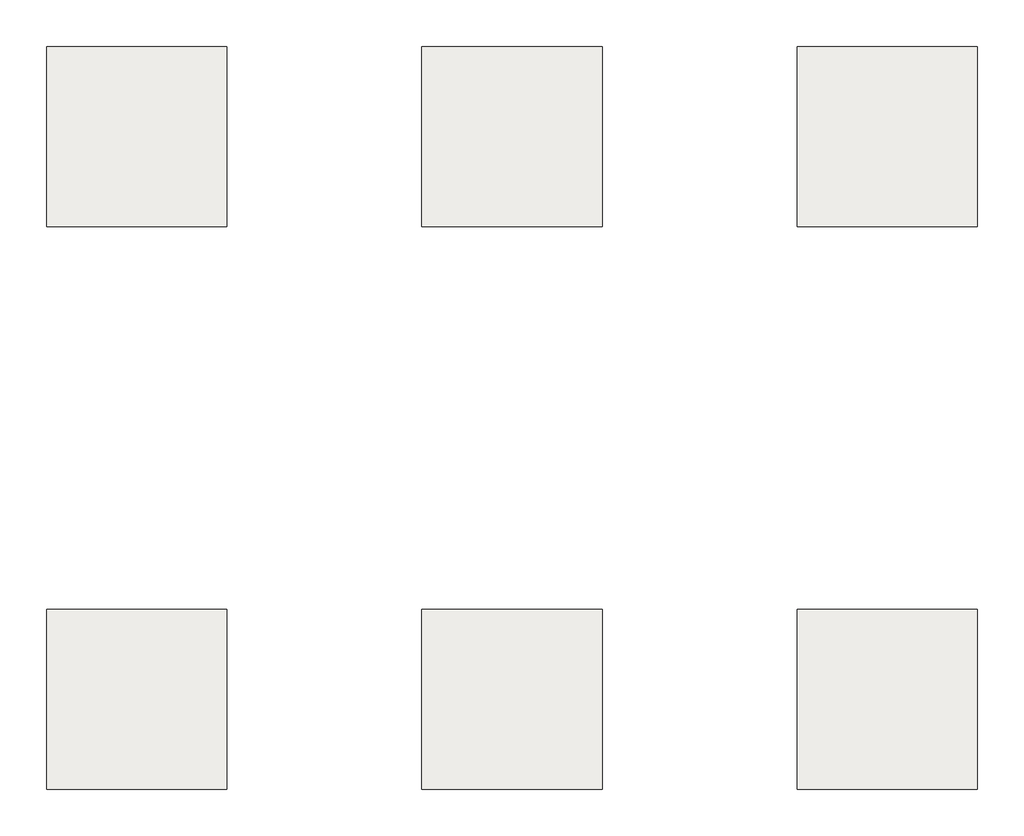
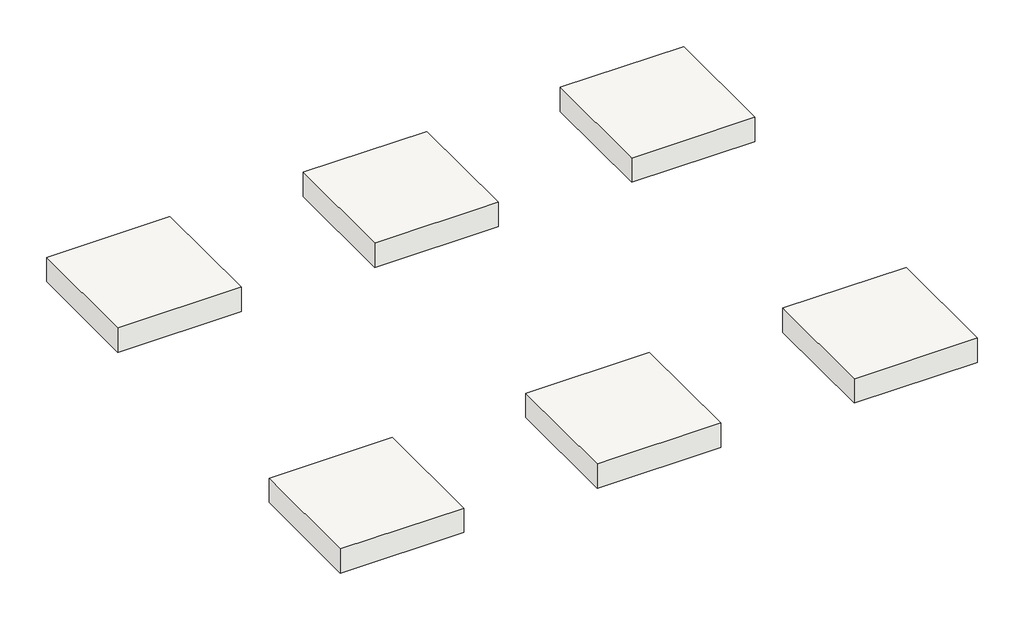
# Not in any storey: 6 slabs.
"""IFC4 building model written with IfcOpenShell, lengths in millimetres."""

import ifcopenshell
import ifcopenshell.guid

model = None  # the IFC model being written
_history = None  # IfcOwnerHistory: only IFC2X3 demands one
_inside = {}  # id of a spatial element -> (the spatial element, [elements in it])
_under = {}  # id of a project, library or spatial element -> (it, [spatial elements below it])
_declared = {}  # id of a project -> (the project, [libraries it declares])
_typed = {}  # id of a type object -> (the type object, [elements of that type])
_made_of = {}  # id of a material, layer set ... -> (it, [elements and type objects made of it])


def new_model(schema):
    """Start an empty IFC model of exactly this schema.

    Asked for "IFC4X3", IfcOpenShell would pick the latest addendum, in which some entities
    have other attributes; the version numbers below select the first issue.
    IFC2X3 requires an IfcOwnerHistory on every rooted entity: one is made here for all.
    """
    global model, _history
    if schema == "IFC4X3":
        model = ifcopenshell.file(schema_version=(4, 3, 0, 0))
    else:
        model = ifcopenshell.file(schema=schema)
    _inside.clear()
    _under.clear()
    _declared.clear()
    _typed.clear()
    _made_of.clear()
    _history = None
    if model.schema == "IFC2X3":
        org = make("IfcOrganization", Name="unknown")
        user = make(
            "IfcPersonAndOrganization",
            ThePerson=make("IfcPerson", FamilyName="unknown"),
            TheOrganization=org,
        )
        app = make(
            "IfcApplication",
            ApplicationDeveloper=org,
            Version="unknown",
            ApplicationFullName="unknown",
            ApplicationIdentifier="unknown",
        )
        _history = make(
            "IfcOwnerHistory",
            OwningUser=user,
            OwningApplication=app,
            ChangeAction="ADDED",
            CreationDate=0,
        )
    return model


def make(cls, **values):
    """One entity of the class cls with the attributes given. An attribute that is None is left unset."""
    return model.create_entity(
        cls, **{name: value for name, value in values.items() if value is not None}
    )


def rooted(cls, **values):
    """An entity with a GlobalId (a new one), such as an element, a storey or a relation."""
    return make(cls, GlobalId=ifcopenshell.guid.new(), OwnerHistory=_history, **values)


def si_unit(unit_type, name, prefix=None):
    """IfcSIUnit, for example si_unit("LENGTHUNIT", "METRE", prefix="MILLI")."""
    return make("IfcSIUnit", UnitType=unit_type, Prefix=prefix, Name=name)


def assignment(units):
    """IfcUnitAssignment: the units of a project."""
    return None if units is None else make("IfcUnitAssignment", Units=units)


def point(xyz):
    """IfcCartesianPoint."""
    return None if xyz is None else make("IfcCartesianPoint", Coordinates=xyz)


def direction(xyz):
    """IfcDirection."""
    return None if xyz is None else make("IfcDirection", DirectionRatios=xyz)


def frame(location, z_axis=None, x_axis=None):
    """IfcAxis2Placement3D, a coordinate frame: its origin and axes. An axis left out is left unset."""
    return make(
        "IfcAxis2Placement3D",
        Location=point(location),
        Axis=direction(z_axis),
        RefDirection=direction(x_axis),
    )


def origin():
    """The frame at (0, 0, 0) with its axes left unset."""
    return frame((0.0, 0.0, 0.0))


def place(relative_to, where):
    """IfcLocalPlacement: puts the frame where relative to a parent placement (None: the world)."""
    return make(
        "IfcLocalPlacement", PlacementRelTo=relative_to, RelativePlacement=where
    )


def context(
    kind, dimensions, precision=None, world=None, true_north=None, identifier=None
):
    """IfcGeometricRepresentationContext, for example the 3D "Model" context."""
    return make(
        "IfcGeometricRepresentationContext",
        ContextIdentifier=identifier,
        ContextType=kind,
        CoordinateSpaceDimension=dimensions,
        Precision=precision,
        WorldCoordinateSystem=world,
        TrueNorth=true_north,
    )


def project(units=None, contexts=None):
    """IfcProject with its units and contexts."""
    return rooted(
        "IfcProject",
        Name="project",
        RepresentationContexts=contexts,
        UnitsInContext=assignment(units),
    )


def spatial(cls, under=None, at=None, **own):
    """A site, building, storey or space (cls), placed at a placement, below another one or the project."""
    s = rooted(cls, ObjectPlacement=at, **own)
    if under is not None:
        _under.setdefault(under.id(), (under, []))[1].append(s)
    return s


def polyline(points):
    """IfcPolyline through the points."""
    return make("IfcPolyline", Points=[point(p) for p in points])


def outline(outer, holes=None, kind="AREA"):
    """IfcArbitraryClosedProfileDef: a profile drawn as a closed curve; with holes, ...WithVoids."""
    if holes is None:
        return make("IfcArbitraryClosedProfileDef", ProfileType=kind, OuterCurve=outer)
    return make(
        "IfcArbitraryProfileDefWithVoids",
        ProfileType=kind,
        OuterCurve=outer,
        InnerCurves=holes,
    )


def extrude(swept, where, along, depth):
    """IfcExtrudedAreaSolid: the profile swept, set in the frame where, extruded along a direction by depth."""
    return make(
        "IfcExtrudedAreaSolid",
        SweptArea=swept,
        Position=where,
        ExtrudedDirection=direction(along),
        Depth=depth,
    )


def shape(context_of_items, identifier, shape_type, items):
    """IfcShapeRepresentation: the items that make up one representation, for example the "Body"."""
    return make(
        "IfcShapeRepresentation",
        ContextOfItems=context_of_items,
        RepresentationIdentifier=identifier,
        RepresentationType=shape_type,
        Items=items,
    )


def source(mapping_origin, context_of_items, identifier, shape_type, items):
    """IfcRepresentationMap: a shape defined once, which mapped items show again and again."""
    return make(
        "IfcRepresentationMap",
        MappingOrigin=mapping_origin,
        MappedRepresentation=shape(context_of_items, identifier, shape_type, items),
    )


def transform(
    local_origin,
    x_axis=None,
    y_axis=None,
    z_axis=None,
    scale=None,
    scale2=None,
    scale3=None,
    uniform=True,
):
    """IfcCartesianTransformationOperator3D, or its non-uniform kind. x_axis, y_axis, z_axis: its Axis1, 2, 3."""
    if uniform:
        return make(
            "IfcCartesianTransformationOperator3D",
            Axis1=direction(x_axis),
            Axis2=direction(y_axis),
            LocalOrigin=point(local_origin),
            Scale=scale,
            Axis3=direction(z_axis),
        )
    return make(
        "IfcCartesianTransformationOperator3DnonUniform",
        Axis1=direction(x_axis),
        Axis2=direction(y_axis),
        LocalOrigin=point(local_origin),
        Scale=scale,
        Axis3=direction(z_axis),
        Scale2=scale2,
        Scale3=scale3,
    )


def mapped(mapping_source, mapping_target):
    """IfcMappedItem: shows the shape of a source again, moved by a transform."""
    return make(
        "IfcMappedItem", MappingSource=mapping_source, MappingTarget=mapping_target
    )


def made_of(thing, what):
    """Note that an element or type object is made of a material, layer set ...; save() writes the relation."""
    if what is not None:
        _made_of.setdefault(what.id(), (what, []))[1].append(thing)
    return thing


def element(
    cls,
    number,
    at=None,
    inside=None,
    cuts=None,
    type_object=None,
    material=None,
    context=None,
    identifier="Body",
    shape_type=None,
    held_by="IfcProductDefinitionShape",
    body=None,
    shapes=None,
    **own,
):
    """One element of the class cls, such as IfcWall. Its Tag is "e" and its number.

    at: its placement. inside: the storey or other place that contains it. cuts: it is an
    opening in that element (IfcRelVoidsElement). A single representation is given by context,
    identifier, shape_type and body (its items); several are given by shapes. held_by: the class
    of the entity that holds the representations. save() writes the other relations.
    """
    e = rooted(cls, Tag="e%d" % number, ObjectPlacement=at, **own)
    if body is not None:
        shapes = [shape(context, identifier, shape_type, body)]
    if shapes is not None:
        e.Representation = make(held_by, Representations=shapes)
    if inside is not None:
        _inside.setdefault(inside.id(), (inside, []))[1].append(e)
    if cuts is not None:
        rooted(
            "IfcRelVoidsElement", RelatingBuildingElement=cuts, RelatedOpeningElement=e
        )
    if type_object is not None:
        _typed.setdefault(type_object.id(), (type_object, []))[1].append(e)
    return made_of(e, material)


def aggregate(whole, parts):
    """IfcRelAggregates: a whole, such as a stair, and the parts it consists of."""
    return rooted("IfcRelAggregates", RelatingObject=whole, RelatedObjects=parts)


def save(model, path):
    """Write the relations noted so far, then the file.

    IfcRelAggregates (storeys below a building ...), IfcRelContainedInSpatialStructure (elements
    in a storey), IfcRelDefinesByType, IfcRelAssociatesMaterial and IfcRelDeclares: one each for
    every whole, place, type object, material and project.
    """
    for whole, parts in _under.values():
        aggregate(whole, parts)
    for where, things in _inside.values():
        rooted(
            "IfcRelContainedInSpatialStructure",
            RelatedElements=things,
            RelatingStructure=where,
        )
    for kind, things in _typed.values():
        rooted("IfcRelDefinesByType", RelatedObjects=things, RelatingType=kind)
    for what, things in _made_of.values():
        rooted("IfcRelAssociatesMaterial", RelatedObjects=things, RelatingMaterial=what)
    for by, libraries in _declared.values():
        rooted("IfcRelDeclares", RelatingContext=by, RelatedDefinitions=libraries)
    model.write(path)


def foundation_rectangular_non_pile_5fe39465(model_context):
    return source(origin(), model_context, "Body", "SweptSolid", [
        extrude(outline(polyline([(1200.0, 1200.0), (1200.0, -1200.0), (-1200.0, -1200.0), (-1200.0, 1200.0), (1200.0, 1200.0)])), frame((0.0, 0.0, -500.0), z_axis=(0.0, 0.0, 1.0), x_axis=(1.0, 0.0, 0.0)), (0.0, 0.0, 1.0), 500.0),
    ])


model = new_model("IFC4")

# Units and contexts
model_context = context("Model", 3, world=origin())
ifc_project = project(units=[si_unit("LENGTHUNIT", "METRE", prefix="MILLI")], contexts=[model_context])

# Site, building
site = spatial("IfcSite", under=ifc_project)
building = spatial("IfcBuilding", under=site)

# Slabs
placement = place(None, origin())
element("IfcSlab", 1, ObjectType="Foundation Rectangular (Non-Pile) : H_SF_ACF_W2400xL2400xT500", at=placement, inside=building, context=model_context, shape_type="SweptSolid", body=[
    extrude(outline(polyline([(11200.0, 22199.5208589), (11200.0, 19799.5208589), (8800.0, 19799.5208589), (8800.0, 22199.5208589), (11200.0, 22199.5208589)])), frame((0.0, 0.0, -1800.0), z_axis=(0.0, 0.0, 1.0), x_axis=(1.0, 0.0, 0.0)), (0.0, 0.0, 1.0), 500.0),
])
element("IfcSlab", 2, ObjectType="Foundation Rectangular (Non-Pile) : H_SF_ACF_W2400xL2400xT500", at=placement, inside=building, context=model_context, shape_type="SweptSolid", body=[
    extrude(outline(polyline([(6200.0, 22199.5208589), (6200.0, 19799.5208589), (3800.0, 19799.5208589), (3800.0, 22199.5208589), (6200.0, 22199.5208589)])), frame((0.0, 0.0, -1800.0), z_axis=(0.0, 0.0, 1.0), x_axis=(1.0, 0.0, 0.0)), (0.0, 0.0, 1.0), 500.0),
])
element("IfcSlab", 3, ObjectType="Foundation Rectangular (Non-Pile) : H_SF_ACF_W2400xL2400xT500", at=placement, inside=building, context=model_context, shape_type="SweptSolid", body=[
    extrude(outline(polyline([(1200.0, 22199.5208589), (1200.0, 19799.5208589), (-1200.0, 19799.5208589), (-1200.0, 22199.5208589), (1200.0, 22199.5208589)])), frame((0.0, 0.0, -1800.0), z_axis=(0.0, 0.0, 1.0), x_axis=(1.0, 0.0, 0.0)), (0.0, 0.0, 1.0), 500.0),
])
element("IfcSlab", 4, ObjectType="Foundation Rectangular (Non-Pile) : H_SF_ACF_W2400xL2400xT500", at=placement, inside=building, context=model_context, shape_type="SweptSolid", body=[
    extrude(outline(polyline([(1200.0, 14699.5208589), (1200.0, 12299.5208589), (-1200.0, 12299.5208589), (-1200.0, 14699.5208589), (1200.0, 14699.5208589)])), frame((0.0, 0.0, -1800.0), z_axis=(0.0, 0.0, 1.0), x_axis=(1.0, 0.0, 0.0)), (0.0, 0.0, 1.0), 500.0),
])
foundation_rectangular_non_pile_shape = foundation_rectangular_non_pile_5fe39465(model_context)
element("IfcSlab", 5, ObjectType="Foundation Rectangular (Non-Pile) : H_SF_ACF_W2400xL2400xT500", at=placement, inside=building, context=model_context, shape_type="MappedRepresentation", body=[
    mapped(foundation_rectangular_non_pile_shape, transform((5000.0, 13499.5208589, -1300.0), x_axis=(1.0, 0.0, 0.0), y_axis=(0.0, 1.0, 0.0), z_axis=(0.0, 0.0, 1.0))),
])
element("IfcSlab", 6, ObjectType="Foundation Rectangular (Non-Pile) : H_SF_ACF_W2400xL2400xT500", at=placement, inside=building, context=model_context, shape_type="MappedRepresentation", body=[
    mapped(foundation_rectangular_non_pile_shape, transform((10000.0, 13499.5208589, -1300.0), x_axis=(1.0, 0.0, 0.0), y_axis=(0.0, 1.0, 0.0), z_axis=(0.0, 0.0, 1.0))),
])

save(model, "model.ifc")

# Revit data of these elements
# Project information
#   Building Name = "MAIN GATE SECURITY BUILDING"
#   Project Status = "Project Status"
#   Client Name = "현대엔지니어링"
#   Project Address = "서울시 종로구 율곡로 75(계동)"
#   Project Name = "Therma Visayas Energy Project"
#   Project Number = "-"
# Grids (mm)
#   "A": line (0, 24502.793) -> (0, 11308.625)
#   "B": line (5000, 24502.793) -> (5000, 11308.625)
#   "C": line (10000, 24502.793) -> (10000, 11308.625)
#   "1": line (-3860.098, 13499.521) -> (12441.468, 13499.521)
#   "2": line (-3860.098, 20999.521) -> (12441.468, 20999.521)
# Type "Foundation Rectangular (Non-Pile) : H_SF_ACF_W2400xL2400xT500"
#   Top bar = "D25@300"
#   Description = "UG Shallow Foundation"
#   Bottom bar = "D20@300"
#   Width = 2400 mm
#   Length = 2400 mm
#   Foundation Thickness = 500 mm
#   Structural Material [instance default] = A03AC032-00007_Structural Concrete_Type1_25MPa-30Mpa
#   Assembly Code = ""
# Elements 1, 2, 3, 4, 5, 6 (IfcSlab, "Foundation Rectangular (Non-Pile) : H_SF_ACF_W2400xL2400xT500")
#   Comments = ""
#   Mark = "F1"
#   Structural Material = A03AC032-00007_Structural Concrete_Type1_25MPa-30Mpa
#   Phase Created = New Construction
#   Materials on its faces: "A03AC032-00007_Structural Concrete_Type1_25MPa-30Mpa"
# Materials
#   "A03AC032-00007_Structural Concrete_Type1_25MPa-30Mpa": class "Concrete", colour RGB 176 176 176, transparency 0, Keynote = "09910.A1", Description = "Reinf. Conc.", Cost = 0
